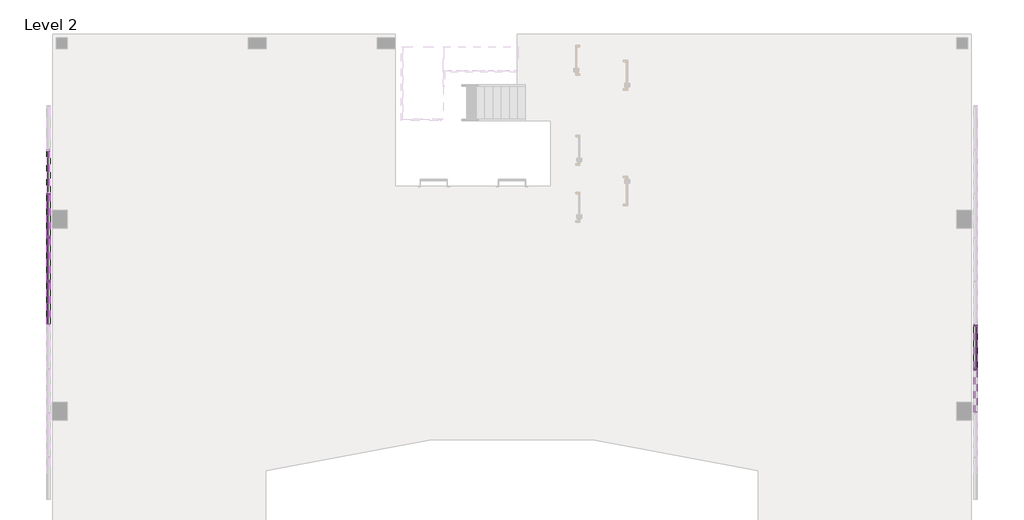
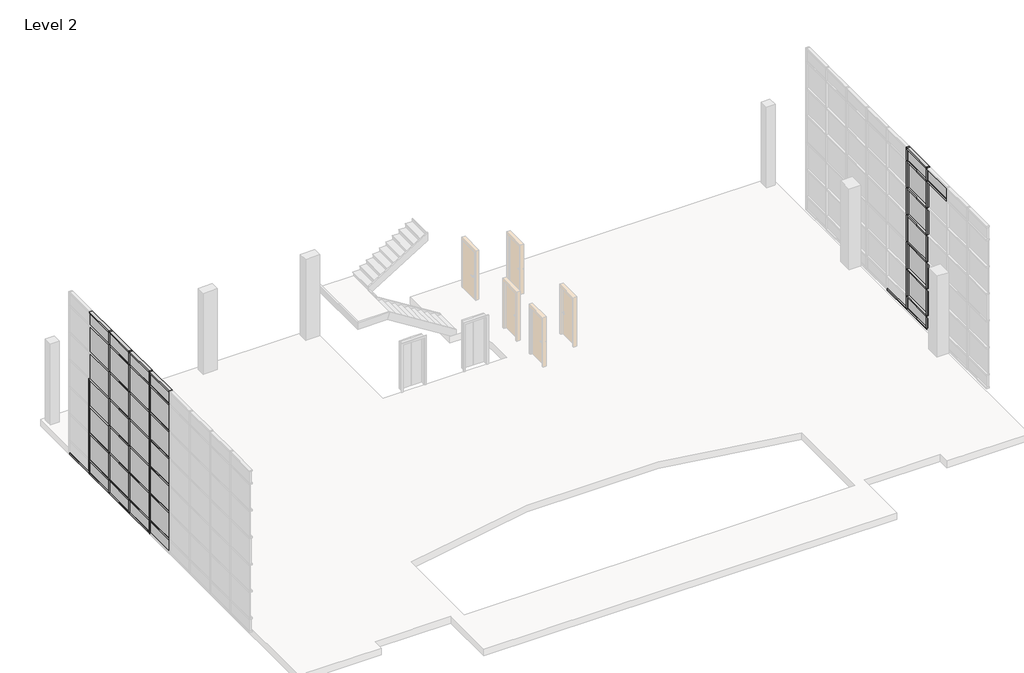
# One storey, part 4 of 6: 77 members, 36 plates.
"""IFC4 building model written with IfcOpenShell, lengths in millimetres."""

import ifcopenshell
import ifcopenshell.guid

model = None  # the IFC model being written
_history = None  # IfcOwnerHistory: only IFC2X3 demands one
_inside = {}  # id of a spatial element -> (the spatial element, [elements in it])
_under = {}  # id of a project, library or spatial element -> (it, [spatial elements below it])
_declared = {}  # id of a project -> (the project, [libraries it declares])
_typed = {}  # id of a type object -> (the type object, [elements of that type])
_made_of = {}  # id of a material, layer set ... -> (it, [elements and type objects made of it])


def new_model(schema):
    """Start an empty IFC model of exactly this schema.

    Asked for "IFC4X3", IfcOpenShell would pick the latest addendum, in which some entities
    have other attributes; the version numbers below select the first issue.
    IFC2X3 requires an IfcOwnerHistory on every rooted entity: one is made here for all.
    """
    global model, _history
    if schema == "IFC4X3":
        model = ifcopenshell.file(schema_version=(4, 3, 0, 0))
    else:
        model = ifcopenshell.file(schema=schema)
    _inside.clear()
    _under.clear()
    _declared.clear()
    _typed.clear()
    _made_of.clear()
    _history = None
    if model.schema == "IFC2X3":
        org = make("IfcOrganization", Name="unknown")
        user = make(
            "IfcPersonAndOrganization",
            ThePerson=make("IfcPerson", FamilyName="unknown"),
            TheOrganization=org,
        )
        app = make(
            "IfcApplication",
            ApplicationDeveloper=org,
            Version="unknown",
            ApplicationFullName="unknown",
            ApplicationIdentifier="unknown",
        )
        _history = make(
            "IfcOwnerHistory",
            OwningUser=user,
            OwningApplication=app,
            ChangeAction="ADDED",
            CreationDate=0,
        )
    return model


def make(cls, **values):
    """One entity of the class cls with the attributes given. An attribute that is None is left unset."""
    return model.create_entity(
        cls, **{name: value for name, value in values.items() if value is not None}
    )


def rooted(cls, **values):
    """An entity with a GlobalId (a new one), such as an element, a storey or a relation."""
    return make(cls, GlobalId=ifcopenshell.guid.new(), OwnerHistory=_history, **values)


def si_unit(unit_type, name, prefix=None):
    """IfcSIUnit, for example si_unit("LENGTHUNIT", "METRE", prefix="MILLI")."""
    return make("IfcSIUnit", UnitType=unit_type, Prefix=prefix, Name=name)


def assignment(units):
    """IfcUnitAssignment: the units of a project."""
    return None if units is None else make("IfcUnitAssignment", Units=units)


def point(xyz):
    """IfcCartesianPoint."""
    return None if xyz is None else make("IfcCartesianPoint", Coordinates=xyz)


def direction(xyz):
    """IfcDirection."""
    return None if xyz is None else make("IfcDirection", DirectionRatios=xyz)


def frame(location, z_axis=None, x_axis=None):
    """IfcAxis2Placement3D, a coordinate frame: its origin and axes. An axis left out is left unset."""
    return make(
        "IfcAxis2Placement3D",
        Location=point(location),
        Axis=direction(z_axis),
        RefDirection=direction(x_axis),
    )


def origin():
    """The frame at (0, 0, 0) with its axes left unset."""
    return frame((0.0, 0.0, 0.0))


def origin_with_axes():
    """The frame at (0, 0, 0) with the z axis (0, 0, 1) and the x axis (1, 0, 0) written out."""
    return frame((0.0, 0.0, 0.0), z_axis=(0.0, 0.0, 1.0), x_axis=(1.0, 0.0, 0.0))


def place(relative_to, where):
    """IfcLocalPlacement: puts the frame where relative to a parent placement (None: the world)."""
    return make(
        "IfcLocalPlacement", PlacementRelTo=relative_to, RelativePlacement=where
    )


def context(
    kind, dimensions, precision=None, world=None, true_north=None, identifier=None
):
    """IfcGeometricRepresentationContext, for example the 3D "Model" context."""
    return make(
        "IfcGeometricRepresentationContext",
        ContextIdentifier=identifier,
        ContextType=kind,
        CoordinateSpaceDimension=dimensions,
        Precision=precision,
        WorldCoordinateSystem=world,
        TrueNorth=true_north,
    )


def project(units=None, contexts=None):
    """IfcProject with its units and contexts."""
    return rooted(
        "IfcProject",
        Name="project",
        RepresentationContexts=contexts,
        UnitsInContext=assignment(units),
    )


def spatial(cls, under=None, at=None, **own):
    """A site, building, storey or space (cls), placed at a placement, below another one or the project."""
    s = rooted(cls, ObjectPlacement=at, **own)
    if under is not None:
        _under.setdefault(under.id(), (under, []))[1].append(s)
    return s


def polyline(points):
    """IfcPolyline through the points."""
    return make("IfcPolyline", Points=[point(p) for p in points])


def outline(outer, holes=None, kind="AREA"):
    """IfcArbitraryClosedProfileDef: a profile drawn as a closed curve; with holes, ...WithVoids."""
    if holes is None:
        return make("IfcArbitraryClosedProfileDef", ProfileType=kind, OuterCurve=outer)
    return make(
        "IfcArbitraryProfileDefWithVoids",
        ProfileType=kind,
        OuterCurve=outer,
        InnerCurves=holes,
    )


def extrude(swept, where, along, depth):
    """IfcExtrudedAreaSolid: the profile swept, set in the frame where, extruded along a direction by depth."""
    return make(
        "IfcExtrudedAreaSolid",
        SweptArea=swept,
        Position=where,
        ExtrudedDirection=direction(along),
        Depth=depth,
    )


def shape(context_of_items, identifier, shape_type, items):
    """IfcShapeRepresentation: the items that make up one representation, for example the "Body"."""
    return make(
        "IfcShapeRepresentation",
        ContextOfItems=context_of_items,
        RepresentationIdentifier=identifier,
        RepresentationType=shape_type,
        Items=items,
    )


def source(mapping_origin, context_of_items, identifier, shape_type, items):
    """IfcRepresentationMap: a shape defined once, which mapped items show again and again."""
    return make(
        "IfcRepresentationMap",
        MappingOrigin=mapping_origin,
        MappedRepresentation=shape(context_of_items, identifier, shape_type, items),
    )


def transform(
    local_origin,
    x_axis=None,
    y_axis=None,
    z_axis=None,
    scale=None,
    scale2=None,
    scale3=None,
    uniform=True,
):
    """IfcCartesianTransformationOperator3D, or its non-uniform kind. x_axis, y_axis, z_axis: its Axis1, 2, 3."""
    if uniform:
        return make(
            "IfcCartesianTransformationOperator3D",
            Axis1=direction(x_axis),
            Axis2=direction(y_axis),
            LocalOrigin=point(local_origin),
            Scale=scale,
            Axis3=direction(z_axis),
        )
    return make(
        "IfcCartesianTransformationOperator3DnonUniform",
        Axis1=direction(x_axis),
        Axis2=direction(y_axis),
        LocalOrigin=point(local_origin),
        Scale=scale,
        Axis3=direction(z_axis),
        Scale2=scale2,
        Scale3=scale3,
    )


def mapped(mapping_source, mapping_target):
    """IfcMappedItem: shows the shape of a source again, moved by a transform."""
    return make(
        "IfcMappedItem", MappingSource=mapping_source, MappingTarget=mapping_target
    )


def made_of(thing, what):
    """Note that an element or type object is made of a material, layer set ...; save() writes the relation."""
    if what is not None:
        _made_of.setdefault(what.id(), (what, []))[1].append(thing)
    return thing


def element(
    cls,
    number,
    at=None,
    inside=None,
    cuts=None,
    type_object=None,
    material=None,
    context=None,
    identifier="Body",
    shape_type=None,
    held_by="IfcProductDefinitionShape",
    body=None,
    shapes=None,
    **own,
):
    """One element of the class cls, such as IfcWall. Its Tag is "e" and its number.

    at: its placement. inside: the storey or other place that contains it. cuts: it is an
    opening in that element (IfcRelVoidsElement). A single representation is given by context,
    identifier, shape_type and body (its items); several are given by shapes. held_by: the class
    of the entity that holds the representations. save() writes the other relations.
    """
    e = rooted(cls, Tag="e%d" % number, ObjectPlacement=at, **own)
    if body is not None:
        shapes = [shape(context, identifier, shape_type, body)]
    if shapes is not None:
        e.Representation = make(held_by, Representations=shapes)
    if inside is not None:
        _inside.setdefault(inside.id(), (inside, []))[1].append(e)
    if cuts is not None:
        rooted(
            "IfcRelVoidsElement", RelatingBuildingElement=cuts, RelatedOpeningElement=e
        )
    if type_object is not None:
        _typed.setdefault(type_object.id(), (type_object, []))[1].append(e)
    return made_of(e, material)


def aggregate(whole, parts):
    """IfcRelAggregates: a whole, such as a stair, and the parts it consists of."""
    return rooted("IfcRelAggregates", RelatingObject=whole, RelatedObjects=parts)


def save(model, path):
    """Write the relations noted so far, then the file.

    IfcRelAggregates (storeys below a building ...), IfcRelContainedInSpatialStructure (elements
    in a storey), IfcRelDefinesByType, IfcRelAssociatesMaterial and IfcRelDeclares: one each for
    every whole, place, type object, material and project.
    """
    for whole, parts in _under.values():
        aggregate(whole, parts)
    for where, things in _inside.values():
        rooted(
            "IfcRelContainedInSpatialStructure",
            RelatedElements=things,
            RelatingStructure=where,
        )
    for kind, things in _typed.values():
        rooted("IfcRelDefinesByType", RelatedObjects=things, RelatingType=kind)
    for what, things in _made_of.values():
        rooted("IfcRelAssociatesMaterial", RelatedObjects=things, RelatingMaterial=what)
    for by, libraries in _declared.values():
        rooted("IfcRelDeclares", RelatingContext=by, RelatedDefinitions=libraries)
    model.write(path)


def member_2e151cea(model_context):
    return source(origin(), model_context, "Body", "SweptSolid", [
        extrude(outline(polyline([(0.0, 63.5), (0.0, -63.5), (-63.5, -63.5), (-63.5, 63.5), (0.0, 63.5)])), frame((0.0, 0.0, -1426.6333333), z_axis=(0.0, 0.0, 1.0), x_axis=(1.0, 0.0, 0.0)), (0.0, 0.0, 1.0), 1426.6333333),
    ])


def member_7b0bb32c(model_context):
    return source(origin(), model_context, "Body", "SweptSolid", [
        extrude(outline(polyline([(0.0, 63.5), (0.0, -63.5), (-63.5, -63.5), (-63.5, 63.5), (0.0, 63.5)])), frame((0.0, 0.0, -1394.8833336), z_axis=(0.0, 0.0, 1.0), x_axis=(1.0, 0.0, 0.0)), (0.0, 0.0, 1.0), 1394.8833336),
    ])


def member_3c30aa5e(model_context):
    return source(origin(), model_context, "Body", "SweptSolid", [
        extrude(outline(polyline([(31.75, 63.5), (31.75, -63.5), (-31.75, -63.5), (-31.75, 63.5), (31.75, 63.5)])), frame((0.0, 0.0, -1426.6333333), z_axis=(0.0, 0.0, 1.0), x_axis=(1.0, 0.0, 0.0)), (0.0, 0.0, 1.0), 1426.6333333),
    ])


def member_2b49869a(model_context):
    return source(origin(), model_context, "Body", "SweptSolid", [
        extrude(outline(polyline([(31.75, 63.5), (31.75, -63.5), (-31.75, -63.5), (-31.75, 63.5), (31.75, 63.5)])), frame((0.0, 0.0, -1219.2), z_axis=(0.0, 0.0, 1.0), x_axis=(1.0, 0.0, 0.0)), (0.0, 0.0, 1.0), 1219.2),
    ])


def member_6e77e263(model_context):
    return source(origin(), model_context, "Body", "SweptSolid", [
        extrude(outline(polyline([(31.75, 63.5), (31.75, -63.5), (-31.75, -63.5), (-31.75, 63.5), (31.75, 63.5)])), frame((0.0, 0.0, -609.6), z_axis=(0.0, 0.0, 1.0), x_axis=(1.0, 0.0, 0.0)), (0.0, 0.0, 1.0), 609.6),
    ])


def system_panel_glazed_8e8b8cb0(model_context):
    return source(origin(), model_context, "Body", "SweptSolid", [
        extrude(outline(polyline([(713.3166666, 19.05), (-713.3166666, 19.05), (-713.3166666, 44.45), (713.3166666, 44.45), (713.3166666, 19.05)])), origin_with_axes(), (0.0, 0.0, 1.0), 1155.7),
    ])


def system_panel_glazed_0adb819a(model_context):
    return source(origin(), model_context, "Body", "SweptSolid", [
        extrude(outline(polyline([(713.3166666, -44.45), (-713.3166666, -44.45), (-713.3166666, -19.05), (713.3166666, -19.05), (713.3166666, -44.45)])), origin_with_axes(), (0.0, 0.0, 1.0), 1155.7),
    ])


def system_panel_solid_81e17396(model_context):
    return source(origin(), model_context, "Body", "SweptSolid", [
        extrude(outline(polyline([(713.3166666, -19.05), (-713.3166666, -19.05), (-713.3166666, 44.45), (713.3166666, 44.45), (713.3166666, -19.05)])), origin_with_axes(), (0.0, 0.0, 1.0), 1155.7),
    ])


def system_panel_solid_4932440a(model_context):
    return source(origin(), model_context, "Body", "SweptSolid", [
        extrude(outline(polyline([(713.3166666, -19.05), (-713.3166666, -19.05), (-713.3166666, 44.45), (713.3166666, 44.45), (713.3166666, -19.05)])), origin_with_axes(), (0.0, 0.0, 1.0), 514.35),
    ])


def system_panel_solid_81598777(model_context):
    return source(origin(), model_context, "Body", "SweptSolid", [
        extrude(outline(polyline([(713.3166666, -44.45), (-713.3166666, -44.45), (-713.3166666, 19.05), (713.3166666, 19.05), (713.3166666, -44.45)])), origin_with_axes(), (0.0, 0.0, 1.0), 514.35),
    ])


def system_panel_solid_db88bede(model_context):
    return source(origin(), model_context, "Body", "SweptSolid", [
        extrude(outline(polyline([(713.3166666, -44.45), (-713.3166666, -44.45), (-713.3166666, 19.05), (713.3166666, 19.05), (713.3166666, -44.45)])), origin_with_axes(), (0.0, 0.0, 1.0), 1155.7),
    ])


model = new_model("IFC4")

# Units and contexts
model_context = context("Model", 3, world=origin())
ifc_project = project(units=[si_unit("LENGTHUNIT", "METRE", prefix="MILLI")], contexts=[model_context])

# Site, building, storey
site = spatial("IfcSite", under=ifc_project)
building = spatial("IfcBuilding", under=site)
storey = spatial("IfcBuildingStorey", under=building, Name="Level 2", Elevation=3657.6)

# Members
placement = place(None, origin())
member_shape = member_2e151cea(model_context)
element("IfcMember", 1, ObjectType="Rectangular Mullion : 2.5\" x 5\" rectangular", at=placement, inside=storey, context=model_context, shape_type="MappedRepresentation", body=[
    mapped(member_shape, transform((-16888.4122732, 962.418197, 10972.8), x_axis=(0.0, 0.0, 1.0), y_axis=(1.0, 0.0, 0.0), z_axis=(0.0, 1.0, 0.0))),
])
element("IfcMember", 2, ObjectType="Rectangular Mullion : 2.5\" x 5\" rectangular", at=placement, inside=storey, context=model_context, shape_type="MappedRepresentation", body=[
    mapped(member_shape, transform((-16888.4122732, 2452.5515303, 10972.8), x_axis=(0.0, 0.0, 1.0), y_axis=(1.0, 0.0, 0.0), z_axis=(0.0, 1.0, 0.0))),
])
element("IfcMember", 3, ObjectType="Rectangular Mullion : 2.5\" x 5\" rectangular", at=placement, inside=storey, context=model_context, shape_type="MappedRepresentation", body=[
    mapped(member_shape, transform((-16888.4122732, 3942.6848636, 10972.8), x_axis=(0.0, 0.0, 1.0), y_axis=(1.0, 0.0, 0.0), z_axis=(0.0, 1.0, 0.0))),
])
element("IfcMember", 4, ObjectType="Rectangular Mullion : 2.5\" x 5\" rectangular", at=placement, inside=storey, context=model_context, shape_type="MappedRepresentation", body=[
    mapped(member_shape, transform((-16888.4122732, 5432.8181968, 10972.8), x_axis=(0.0, 0.0, 1.0), y_axis=(1.0, 0.0, 0.0), z_axis=(0.0, 1.0, 0.0))),
])
member_2_shape = member_7b0bb32c(model_context)
element("IfcMember", 5, ObjectType="Rectangular Mullion : 2.5\" x 5\" rectangular", at=placement, inside=storey, context=model_context, shape_type="MappedRepresentation", body=[
    mapped(member_2_shape, transform((-16888.4122732, 5496.3181968, 3657.6), x_axis=(0.0, 0.0, -1.0), y_axis=(1.0, 0.0, 0.0), z_axis=(0.0, -1.0, 0.0))),
])
element("IfcMember", 6, ObjectType="Rectangular Mullion : 2.5\" x 5\" rectangular", at=placement, inside=storey, context=model_context, shape_type="MappedRepresentation", body=[
    mapped(member_shape, transform((-16888.4122732, 1025.918197, 3657.6), x_axis=(0.0, 0.0, -1.0), y_axis=(1.0, 0.0, 0.0), z_axis=(0.0, -1.0, 0.0))),
])
element("IfcMember", 7, ObjectType="Rectangular Mullion : 2.5\" x 5\" rectangular", at=placement, inside=storey, context=model_context, shape_type="MappedRepresentation", body=[
    mapped(member_shape, transform((-16888.4122732, 2516.0515303, 3657.6), x_axis=(0.0, 0.0, -1.0), y_axis=(1.0, 0.0, 0.0), z_axis=(0.0, -1.0, 0.0))),
])
element("IfcMember", 8, ObjectType="Rectangular Mullion : 2.5\" x 5\" rectangular", at=placement, inside=storey, context=model_context, shape_type="MappedRepresentation", body=[
    mapped(member_shape, transform((-16888.4122732, 4006.1848636, 3657.6), x_axis=(0.0, 0.0, -1.0), y_axis=(1.0, 0.0, 0.0), z_axis=(0.0, -1.0, 0.0))),
])
member_3_shape = member_3c30aa5e(model_context)
element("IfcMember", 9, ObjectType="Rectangular Mullion : 2.5\" x 5\" rectangular", at=placement, inside=storey, context=model_context, shape_type="MappedRepresentation", body=[
    mapped(member_3_shape, transform((-16888.4122732, 962.418197, 4267.2), x_axis=(0.0, 0.0, 1.0), y_axis=(1.0, 0.0, 0.0), z_axis=(0.0, 1.0, 0.0))),
])
element("IfcMember", 10, ObjectType="Rectangular Mullion : 2.5\" x 5\" rectangular", at=placement, inside=storey, context=model_context, shape_type="MappedRepresentation", body=[
    mapped(member_3_shape, transform((-16888.4122732, 2452.5515303, 4267.2), x_axis=(0.0, 0.0, 1.0), y_axis=(1.0, 0.0, 0.0), z_axis=(0.0, 1.0, 0.0))),
])
element("IfcMember", 11, ObjectType="Rectangular Mullion : 2.5\" x 5\" rectangular", at=placement, inside=storey, context=model_context, shape_type="MappedRepresentation", body=[
    mapped(member_3_shape, transform((-16888.4122732, 3942.6848636, 4267.2), x_axis=(0.0, 0.0, 1.0), y_axis=(1.0, 0.0, 0.0), z_axis=(0.0, 1.0, 0.0))),
])
element("IfcMember", 12, ObjectType="Rectangular Mullion : 2.5\" x 5\" rectangular", at=placement, inside=storey, context=model_context, shape_type="MappedRepresentation", body=[
    mapped(member_3_shape, transform((-16888.4122732, 5432.8181968, 4267.2), x_axis=(0.0, 0.0, 1.0), y_axis=(1.0, 0.0, 0.0), z_axis=(0.0, 1.0, 0.0))),
])
element("IfcMember", 13, ObjectType="Rectangular Mullion : 2.5\" x 5\" rectangular", at=placement, inside=storey, context=model_context, shape_type="MappedRepresentation", body=[
    mapped(member_3_shape, transform((-16888.4122732, 962.418197, 5486.4), x_axis=(0.0, 0.0, 1.0), y_axis=(1.0, 0.0, 0.0), z_axis=(0.0, 1.0, 0.0))),
])
element("IfcMember", 14, ObjectType="Rectangular Mullion : 2.5\" x 5\" rectangular", at=placement, inside=storey, context=model_context, shape_type="MappedRepresentation", body=[
    mapped(member_3_shape, transform((-16888.4122732, 2452.5515303, 5486.4), x_axis=(0.0, 0.0, 1.0), y_axis=(1.0, 0.0, 0.0), z_axis=(0.0, 1.0, 0.0))),
])
element("IfcMember", 15, ObjectType="Rectangular Mullion : 2.5\" x 5\" rectangular", at=placement, inside=storey, context=model_context, shape_type="MappedRepresentation", body=[
    mapped(member_3_shape, transform((-16888.4122732, 3942.6848636, 5486.4), x_axis=(0.0, 0.0, 1.0), y_axis=(1.0, 0.0, 0.0), z_axis=(0.0, 1.0, 0.0))),
])
element("IfcMember", 16, ObjectType="Rectangular Mullion : 2.5\" x 5\" rectangular", at=placement, inside=storey, context=model_context, shape_type="MappedRepresentation", body=[
    mapped(member_3_shape, transform((-16888.4122732, 5432.8181968, 5486.4), x_axis=(0.0, 0.0, 1.0), y_axis=(1.0, 0.0, 0.0), z_axis=(0.0, 1.0, 0.0))),
])
element("IfcMember", 17, ObjectType="Rectangular Mullion : 2.5\" x 5\" rectangular", at=placement, inside=storey, context=model_context, shape_type="MappedRepresentation", body=[
    mapped(member_3_shape, transform((-16888.4122732, 962.418197, 6705.6), x_axis=(0.0, 0.0, 1.0), y_axis=(1.0, 0.0, 0.0), z_axis=(0.0, 1.0, 0.0))),
])
element("IfcMember", 18, ObjectType="Rectangular Mullion : 2.5\" x 5\" rectangular", at=placement, inside=storey, context=model_context, shape_type="MappedRepresentation", body=[
    mapped(member_3_shape, transform((-16888.4122732, 2452.5515303, 6705.6), x_axis=(0.0, 0.0, 1.0), y_axis=(1.0, 0.0, 0.0), z_axis=(0.0, 1.0, 0.0))),
])
element("IfcMember", 19, ObjectType="Rectangular Mullion : 2.5\" x 5\" rectangular", at=placement, inside=storey, context=model_context, shape_type="MappedRepresentation", body=[
    mapped(member_3_shape, transform((-16888.4122732, 3942.6848636, 6705.6), x_axis=(0.0, 0.0, 1.0), y_axis=(1.0, 0.0, 0.0), z_axis=(0.0, 1.0, 0.0))),
])
element("IfcMember", 20, ObjectType="Rectangular Mullion : 2.5\" x 5\" rectangular", at=placement, inside=storey, context=model_context, shape_type="MappedRepresentation", body=[
    mapped(member_3_shape, transform((-16888.4122732, 962.418197, 7924.8), x_axis=(0.0, 0.0, 1.0), y_axis=(1.0, 0.0, 0.0), z_axis=(0.0, 1.0, 0.0))),
])
element("IfcMember", 21, ObjectType="Rectangular Mullion : 2.5\" x 5\" rectangular", at=placement, inside=storey, context=model_context, shape_type="MappedRepresentation", body=[
    mapped(member_3_shape, transform((-16888.4122732, 2452.5515303, 7924.8), x_axis=(0.0, 0.0, 1.0), y_axis=(1.0, 0.0, 0.0), z_axis=(0.0, 1.0, 0.0))),
])
element("IfcMember", 22, ObjectType="Rectangular Mullion : 2.5\" x 5\" rectangular", at=placement, inside=storey, context=model_context, shape_type="MappedRepresentation", body=[
    mapped(member_3_shape, transform((-16888.4122732, 3942.6848636, 7924.8), x_axis=(0.0, 0.0, 1.0), y_axis=(1.0, 0.0, 0.0), z_axis=(0.0, 1.0, 0.0))),
])
element("IfcMember", 23, ObjectType="Rectangular Mullion : 2.5\" x 5\" rectangular", at=placement, inside=storey, context=model_context, shape_type="MappedRepresentation", body=[
    mapped(member_3_shape, transform((-16888.4122732, 962.418197, 9144.0), x_axis=(0.0, 0.0, 1.0), y_axis=(1.0, 0.0, 0.0), z_axis=(0.0, 1.0, 0.0))),
])
element("IfcMember", 24, ObjectType="Rectangular Mullion : 2.5\" x 5\" rectangular", at=placement, inside=storey, context=model_context, shape_type="MappedRepresentation", body=[
    mapped(member_3_shape, transform((-16888.4122732, 2452.5515303, 9144.0), x_axis=(0.0, 0.0, 1.0), y_axis=(1.0, 0.0, 0.0), z_axis=(0.0, 1.0, 0.0))),
])
element("IfcMember", 25, ObjectType="Rectangular Mullion : 2.5\" x 5\" rectangular", at=placement, inside=storey, context=model_context, shape_type="MappedRepresentation", body=[
    mapped(member_3_shape, transform((-16888.4122732, 3942.6848636, 9144.0), x_axis=(0.0, 0.0, 1.0), y_axis=(1.0, 0.0, 0.0), z_axis=(0.0, 1.0, 0.0))),
])
element("IfcMember", 26, ObjectType="Rectangular Mullion : 2.5\" x 5\" rectangular", at=placement, inside=storey, context=model_context, shape_type="MappedRepresentation", body=[
    mapped(member_3_shape, transform((-16888.4122732, 962.418197, 10363.2), x_axis=(0.0, 0.0, 1.0), y_axis=(1.0, 0.0, 0.0), z_axis=(0.0, 1.0, 0.0))),
])
element("IfcMember", 27, ObjectType="Rectangular Mullion : 2.5\" x 5\" rectangular", at=placement, inside=storey, context=model_context, shape_type="MappedRepresentation", body=[
    mapped(member_3_shape, transform((-16888.4122732, 2452.5515303, 10363.2), x_axis=(0.0, 0.0, 1.0), y_axis=(1.0, 0.0, 0.0), z_axis=(0.0, 1.0, 0.0))),
])
element("IfcMember", 28, ObjectType="Rectangular Mullion : 2.5\" x 5\" rectangular", at=placement, inside=storey, context=model_context, shape_type="MappedRepresentation", body=[
    mapped(member_3_shape, transform((-16888.4122732, 3942.6848636, 10363.2), x_axis=(0.0, 0.0, 1.0), y_axis=(1.0, 0.0, 0.0), z_axis=(0.0, 1.0, 0.0))),
])
member_4_shape = member_2b49869a(model_context)
element("IfcMember", 29, ObjectType="Rectangular Mullion : 2.5\" x 5\" rectangular", at=placement, inside=storey, context=model_context, shape_type="MappedRepresentation", body=[
    mapped(member_4_shape, transform((-16888.4122732, 994.168197, 4267.2), x_axis=(0.0, 1.0, 0.0), y_axis=(1.0, 0.0, 0.0), z_axis=(0.0, 0.0, -1.0))),
])
element("IfcMember", 30, ObjectType="Rectangular Mullion : 2.5\" x 5\" rectangular", at=placement, inside=storey, context=model_context, shape_type="MappedRepresentation", body=[
    mapped(member_4_shape, transform((-16888.4122732, 2484.3015303, 4267.2), x_axis=(0.0, 1.0, 0.0), y_axis=(1.0, 0.0, 0.0), z_axis=(0.0, 0.0, -1.0))),
])
element("IfcMember", 31, ObjectType="Rectangular Mullion : 2.5\" x 5\" rectangular", at=placement, inside=storey, context=model_context, shape_type="MappedRepresentation", body=[
    mapped(member_4_shape, transform((-16888.4122732, 3974.4348636, 4267.2), x_axis=(0.0, 1.0, 0.0), y_axis=(1.0, 0.0, 0.0), z_axis=(0.0, 0.0, -1.0))),
])
element("IfcMember", 32, ObjectType="Rectangular Mullion : 2.5\" x 5\" rectangular", at=placement, inside=storey, context=model_context, shape_type="MappedRepresentation", body=[
    mapped(member_4_shape, transform((-16888.4122732, 5464.5681968, 4267.2), x_axis=(0.0, 1.0, 0.0), y_axis=(1.0, 0.0, 0.0), z_axis=(0.0, 0.0, -1.0))),
])
element("IfcMember", 33, ObjectType="Rectangular Mullion : 2.5\" x 5\" rectangular", at=placement, inside=storey, context=model_context, shape_type="MappedRepresentation", body=[
    mapped(member_4_shape, transform((-16888.4122732, 994.168197, 5486.4), x_axis=(0.0, 1.0, 0.0), y_axis=(1.0, 0.0, 0.0), z_axis=(0.0, 0.0, -1.0))),
])
element("IfcMember", 34, ObjectType="Rectangular Mullion : 2.5\" x 5\" rectangular", at=placement, inside=storey, context=model_context, shape_type="MappedRepresentation", body=[
    mapped(member_4_shape, transform((-16888.4122732, 2484.3015303, 5486.4), x_axis=(0.0, 1.0, 0.0), y_axis=(1.0, 0.0, 0.0), z_axis=(0.0, 0.0, -1.0))),
])
element("IfcMember", 35, ObjectType="Rectangular Mullion : 2.5\" x 5\" rectangular", at=placement, inside=storey, context=model_context, shape_type="MappedRepresentation", body=[
    mapped(member_4_shape, transform((-16888.4122732, 3974.4348636, 5486.4), x_axis=(0.0, 1.0, 0.0), y_axis=(1.0, 0.0, 0.0), z_axis=(0.0, 0.0, -1.0))),
])
element("IfcMember", 36, ObjectType="Rectangular Mullion : 2.5\" x 5\" rectangular", at=placement, inside=storey, context=model_context, shape_type="MappedRepresentation", body=[
    mapped(member_4_shape, transform((-16888.4122732, 5464.5681968, 5486.4), x_axis=(0.0, 1.0, 0.0), y_axis=(1.0, 0.0, 0.0), z_axis=(0.0, 0.0, -1.0))),
])
element("IfcMember", 37, ObjectType="Rectangular Mullion : 2.5\" x 5\" rectangular", at=placement, inside=storey, context=model_context, shape_type="MappedRepresentation", body=[
    mapped(member_4_shape, transform((-16888.4122732, 994.168197, 6705.6), x_axis=(0.0, 1.0, 0.0), y_axis=(1.0, 0.0, 0.0), z_axis=(0.0, 0.0, -1.0))),
])
element("IfcMember", 38, ObjectType="Rectangular Mullion : 2.5\" x 5\" rectangular", at=placement, inside=storey, context=model_context, shape_type="MappedRepresentation", body=[
    mapped(member_4_shape, transform((-16888.4122732, 994.168197, 7924.8), x_axis=(0.0, 1.0, 0.0), y_axis=(1.0, 0.0, 0.0), z_axis=(0.0, 0.0, -1.0))),
])
element("IfcMember", 39, ObjectType="Rectangular Mullion : 2.5\" x 5\" rectangular", at=placement, inside=storey, context=model_context, shape_type="MappedRepresentation", body=[
    mapped(member_4_shape, transform((-16888.4122732, 994.168197, 9144.0), x_axis=(0.0, 1.0, 0.0), y_axis=(1.0, 0.0, 0.0), z_axis=(0.0, 0.0, -1.0))),
])
element("IfcMember", 40, ObjectType="Rectangular Mullion : 2.5\" x 5\" rectangular", at=placement, inside=storey, context=model_context, shape_type="MappedRepresentation", body=[
    mapped(member_4_shape, transform((-16888.4122732, 2484.3015303, 6705.6), x_axis=(0.0, 1.0, 0.0), y_axis=(1.0, 0.0, 0.0), z_axis=(0.0, 0.0, -1.0))),
])
element("IfcMember", 41, ObjectType="Rectangular Mullion : 2.5\" x 5\" rectangular", at=placement, inside=storey, context=model_context, shape_type="MappedRepresentation", body=[
    mapped(member_4_shape, transform((-16888.4122732, 2484.3015303, 7924.8), x_axis=(0.0, 1.0, 0.0), y_axis=(1.0, 0.0, 0.0), z_axis=(0.0, 0.0, -1.0))),
])
element("IfcMember", 42, ObjectType="Rectangular Mullion : 2.5\" x 5\" rectangular", at=placement, inside=storey, context=model_context, shape_type="MappedRepresentation", body=[
    mapped(member_4_shape, transform((-16888.4122732, 2484.3015303, 9144.0), x_axis=(0.0, 1.0, 0.0), y_axis=(1.0, 0.0, 0.0), z_axis=(0.0, 0.0, -1.0))),
])
element("IfcMember", 43, ObjectType="Rectangular Mullion : 2.5\" x 5\" rectangular", at=placement, inside=storey, context=model_context, shape_type="MappedRepresentation", body=[
    mapped(member_4_shape, transform((-16888.4122732, 3974.4348636, 6705.6), x_axis=(0.0, 1.0, 0.0), y_axis=(1.0, 0.0, 0.0), z_axis=(0.0, 0.0, -1.0))),
])
element("IfcMember", 44, ObjectType="Rectangular Mullion : 2.5\" x 5\" rectangular", at=placement, inside=storey, context=model_context, shape_type="MappedRepresentation", body=[
    mapped(member_4_shape, transform((-16888.4122732, 3974.4348636, 7924.8), x_axis=(0.0, 1.0, 0.0), y_axis=(1.0, 0.0, 0.0), z_axis=(0.0, 0.0, -1.0))),
])
element("IfcMember", 45, ObjectType="Rectangular Mullion : 2.5\" x 5\" rectangular", at=placement, inside=storey, context=model_context, shape_type="MappedRepresentation", body=[
    mapped(member_4_shape, transform((-16888.4122732, 3974.4348636, 9144.0), x_axis=(0.0, 1.0, 0.0), y_axis=(1.0, 0.0, 0.0), z_axis=(0.0, 0.0, -1.0))),
])
element("IfcMember", 46, ObjectType="Rectangular Mullion : 2.5\" x 5\" rectangular", at=placement, inside=storey, context=model_context, shape_type="MappedRepresentation", body=[
    mapped(member_4_shape, transform((-16888.4122732, 5464.5681968, 6705.6), x_axis=(0.0, 1.0, 0.0), y_axis=(1.0, 0.0, 0.0), z_axis=(0.0, 0.0, -1.0))),
])
member_5_shape = member_6e77e263(model_context)
element("IfcMember", 47, ObjectType="Rectangular Mullion : 2.5\" x 5\" rectangular", at=placement, inside=storey, context=model_context, shape_type="MappedRepresentation", body=[
    mapped(member_5_shape, transform((-16888.4122732, 994.168197, 3657.6), x_axis=(0.0, 1.0, 0.0), y_axis=(1.0, 0.0, 0.0), z_axis=(0.0, 0.0, -1.0))),
])
element("IfcMember", 48, ObjectType="Rectangular Mullion : 2.5\" x 5\" rectangular", at=placement, inside=storey, context=model_context, shape_type="MappedRepresentation", body=[
    mapped(member_5_shape, transform((-16888.4122732, 2484.3015303, 3657.6), x_axis=(0.0, 1.0, 0.0), y_axis=(1.0, 0.0, 0.0), z_axis=(0.0, 0.0, -1.0))),
])
element("IfcMember", 49, ObjectType="Rectangular Mullion : 2.5\" x 5\" rectangular", at=placement, inside=storey, context=model_context, shape_type="MappedRepresentation", body=[
    mapped(member_5_shape, transform((-16888.4122732, 3974.4348636, 3657.6), x_axis=(0.0, 1.0, 0.0), y_axis=(1.0, 0.0, 0.0), z_axis=(0.0, 0.0, -1.0))),
])
element("IfcMember", 50, ObjectType="Rectangular Mullion : 2.5\" x 5\" rectangular", at=placement, inside=storey, context=model_context, shape_type="MappedRepresentation", body=[
    mapped(member_5_shape, transform((-16888.4122732, 5464.5681968, 3657.6), x_axis=(0.0, 1.0, 0.0), y_axis=(1.0, 0.0, 0.0), z_axis=(0.0, 0.0, -1.0))),
])
element("IfcMember", 51, ObjectType="Rectangular Mullion : 2.5\" x 5\" rectangular", at=placement, inside=storey, context=model_context, shape_type="MappedRepresentation", body=[
    mapped(member_5_shape, transform((-16888.4122732, 994.168197, 10363.2), x_axis=(0.0, 1.0, 0.0), y_axis=(1.0, 0.0, 0.0), z_axis=(0.0, 0.0, -1.0))),
])
element("IfcMember", 52, ObjectType="Rectangular Mullion : 2.5\" x 5\" rectangular", at=placement, inside=storey, context=model_context, shape_type="MappedRepresentation", body=[
    mapped(member_5_shape, transform((-16888.4122732, 2484.3015303, 10363.2), x_axis=(0.0, 1.0, 0.0), y_axis=(1.0, 0.0, 0.0), z_axis=(0.0, 0.0, -1.0))),
])
element("IfcMember", 53, ObjectType="Rectangular Mullion : 2.5\" x 5\" rectangular", at=placement, inside=storey, context=model_context, shape_type="MappedRepresentation", body=[
    mapped(member_5_shape, transform((-16888.4122732, 3974.4348636, 10363.2), x_axis=(0.0, 1.0, 0.0), y_axis=(1.0, 0.0, 0.0), z_axis=(0.0, 0.0, -1.0))),
])
element("IfcMember", 54, ObjectType="Rectangular Mullion : 2.5\" x 5\" rectangular", at=placement, inside=storey, context=model_context, shape_type="MappedRepresentation", body=[
    mapped(member_shape, transform((14556.9638541, -527.7151362, 10972.8), x_axis=(0.0, 0.0, 1.0), y_axis=(1.0, 0.0, 0.0), z_axis=(0.0, 1.0, 0.0))),
])
element("IfcMember", 55, ObjectType="Rectangular Mullion : 2.5\" x 5\" rectangular", at=placement, inside=storey, context=model_context, shape_type="MappedRepresentation", body=[
    mapped(member_shape, transform((14556.9638541, -1954.3484695, 3657.6), x_axis=(0.0, 0.0, -1.0), y_axis=(1.0, 0.0, 0.0), z_axis=(0.0, -1.0, 0.0))),
])
element("IfcMember", 56, ObjectType="Rectangular Mullion : 2.5\" x 5\" rectangular", at=placement, inside=storey, context=model_context, shape_type="MappedRepresentation", body=[
    mapped(member_shape, transform((14556.9638541, -464.2151362, 3657.6), x_axis=(0.0, 0.0, -1.0), y_axis=(1.0, 0.0, 0.0), z_axis=(0.0, -1.0, 0.0))),
])
element("IfcMember", 57, ObjectType="Rectangular Mullion : 2.5\" x 5\" rectangular", at=placement, inside=storey, context=model_context, shape_type="MappedRepresentation", body=[
    mapped(member_3_shape, transform((14556.9638541, -527.7151362, 4267.2), x_axis=(0.0, 0.0, 1.0), y_axis=(1.0, 0.0, 0.0), z_axis=(0.0, 1.0, 0.0))),
])
element("IfcMember", 58, ObjectType="Rectangular Mullion : 2.5\" x 5\" rectangular", at=placement, inside=storey, context=model_context, shape_type="MappedRepresentation", body=[
    mapped(member_3_shape, transform((14556.9638541, -527.7151362, 5486.4), x_axis=(0.0, 0.0, 1.0), y_axis=(1.0, 0.0, 0.0), z_axis=(0.0, 1.0, 0.0))),
])
element("IfcMember", 59, ObjectType="Rectangular Mullion : 2.5\" x 5\" rectangular", at=placement, inside=storey, context=model_context, shape_type="MappedRepresentation", body=[
    mapped(member_3_shape, transform((14556.9638541, -527.7151362, 6705.6), x_axis=(0.0, 0.0, 1.0), y_axis=(1.0, 0.0, 0.0), z_axis=(0.0, 1.0, 0.0))),
])
element("IfcMember", 60, ObjectType="Rectangular Mullion : 2.5\" x 5\" rectangular", at=placement, inside=storey, context=model_context, shape_type="MappedRepresentation", body=[
    mapped(member_3_shape, transform((14556.9638541, -527.7151362, 7924.8), x_axis=(0.0, 0.0, 1.0), y_axis=(1.0, 0.0, 0.0), z_axis=(0.0, 1.0, 0.0))),
])
element("IfcMember", 61, ObjectType="Rectangular Mullion : 2.5\" x 5\" rectangular", at=placement, inside=storey, context=model_context, shape_type="MappedRepresentation", body=[
    mapped(member_3_shape, transform((14556.9638541, -527.7151362, 9144.0), x_axis=(0.0, 0.0, 1.0), y_axis=(1.0, 0.0, 0.0), z_axis=(0.0, 1.0, 0.0))),
])
element("IfcMember", 62, ObjectType="Rectangular Mullion : 2.5\" x 5\" rectangular", at=placement, inside=storey, context=model_context, shape_type="MappedRepresentation", body=[
    mapped(member_3_shape, transform((14556.9638541, -2017.8484695, 10363.2), x_axis=(0.0, 0.0, 1.0), y_axis=(1.0, 0.0, 0.0), z_axis=(0.0, 1.0, 0.0))),
])
element("IfcMember", 63, ObjectType="Rectangular Mullion : 2.5\" x 5\" rectangular", at=placement, inside=storey, context=model_context, shape_type="MappedRepresentation", body=[
    mapped(member_3_shape, transform((14556.9638541, -527.7151362, 10363.2), x_axis=(0.0, 0.0, 1.0), y_axis=(1.0, 0.0, 0.0), z_axis=(0.0, 1.0, 0.0))),
])
element("IfcMember", 64, ObjectType="Rectangular Mullion : 2.5\" x 5\" rectangular", at=placement, inside=storey, context=model_context, shape_type="MappedRepresentation", body=[
    mapped(member_5_shape, transform((14556.9638541, -1986.0984695, 3657.6), x_axis=(0.0, 1.0, 0.0), y_axis=(1.0, 0.0, 0.0), z_axis=(0.0, 0.0, -1.0))),
])
element("IfcMember", 65, ObjectType="Rectangular Mullion : 2.5\" x 5\" rectangular", at=placement, inside=storey, context=model_context, shape_type="MappedRepresentation", body=[
    mapped(member_5_shape, transform((14556.9638541, -495.9651362, 3657.6), x_axis=(0.0, 1.0, 0.0), y_axis=(1.0, 0.0, 0.0), z_axis=(0.0, 0.0, -1.0))),
])
element("IfcMember", 66, ObjectType="Rectangular Mullion : 2.5\" x 5\" rectangular", at=placement, inside=storey, context=model_context, shape_type="MappedRepresentation", body=[
    mapped(member_4_shape, transform((14556.9638541, -1986.0984695, 4267.2), x_axis=(0.0, 1.0, 0.0), y_axis=(1.0, 0.0, 0.0), z_axis=(0.0, 0.0, -1.0))),
])
element("IfcMember", 67, ObjectType="Rectangular Mullion : 2.5\" x 5\" rectangular", at=placement, inside=storey, context=model_context, shape_type="MappedRepresentation", body=[
    mapped(member_4_shape, transform((14556.9638541, -495.9651362, 4267.2), x_axis=(0.0, 1.0, 0.0), y_axis=(1.0, 0.0, 0.0), z_axis=(0.0, 0.0, -1.0))),
])
element("IfcMember", 68, ObjectType="Rectangular Mullion : 2.5\" x 5\" rectangular", at=placement, inside=storey, context=model_context, shape_type="MappedRepresentation", body=[
    mapped(member_4_shape, transform((14556.9638541, -1986.0984695, 5486.4), x_axis=(0.0, 1.0, 0.0), y_axis=(1.0, 0.0, 0.0), z_axis=(0.0, 0.0, -1.0))),
])
element("IfcMember", 69, ObjectType="Rectangular Mullion : 2.5\" x 5\" rectangular", at=placement, inside=storey, context=model_context, shape_type="MappedRepresentation", body=[
    mapped(member_4_shape, transform((14556.9638541, -495.9651362, 5486.4), x_axis=(0.0, 1.0, 0.0), y_axis=(1.0, 0.0, 0.0), z_axis=(0.0, 0.0, -1.0))),
])
element("IfcMember", 70, ObjectType="Rectangular Mullion : 2.5\" x 5\" rectangular", at=placement, inside=storey, context=model_context, shape_type="MappedRepresentation", body=[
    mapped(member_4_shape, transform((14556.9638541, -1986.0984695, 6705.6), x_axis=(0.0, 1.0, 0.0), y_axis=(1.0, 0.0, 0.0), z_axis=(0.0, 0.0, -1.0))),
])
element("IfcMember", 71, ObjectType="Rectangular Mullion : 2.5\" x 5\" rectangular", at=placement, inside=storey, context=model_context, shape_type="MappedRepresentation", body=[
    mapped(member_4_shape, transform((14556.9638541, -1986.0984695, 7924.8), x_axis=(0.0, 1.0, 0.0), y_axis=(1.0, 0.0, 0.0), z_axis=(0.0, 0.0, -1.0))),
])
element("IfcMember", 72, ObjectType="Rectangular Mullion : 2.5\" x 5\" rectangular", at=placement, inside=storey, context=model_context, shape_type="MappedRepresentation", body=[
    mapped(member_4_shape, transform((14556.9638541, -1986.0984695, 9144.0), x_axis=(0.0, 1.0, 0.0), y_axis=(1.0, 0.0, 0.0), z_axis=(0.0, 0.0, -1.0))),
])
element("IfcMember", 73, ObjectType="Rectangular Mullion : 2.5\" x 5\" rectangular", at=placement, inside=storey, context=model_context, shape_type="MappedRepresentation", body=[
    mapped(member_4_shape, transform((14556.9638541, -495.9651362, 6705.6), x_axis=(0.0, 1.0, 0.0), y_axis=(1.0, 0.0, 0.0), z_axis=(0.0, 0.0, -1.0))),
])
element("IfcMember", 74, ObjectType="Rectangular Mullion : 2.5\" x 5\" rectangular", at=placement, inside=storey, context=model_context, shape_type="MappedRepresentation", body=[
    mapped(member_4_shape, transform((14556.9638541, -495.9651362, 7924.8), x_axis=(0.0, 1.0, 0.0), y_axis=(1.0, 0.0, 0.0), z_axis=(0.0, 0.0, -1.0))),
])
element("IfcMember", 75, ObjectType="Rectangular Mullion : 2.5\" x 5\" rectangular", at=placement, inside=storey, context=model_context, shape_type="MappedRepresentation", body=[
    mapped(member_4_shape, transform((14556.9638541, -495.9651362, 9144.0), x_axis=(0.0, 1.0, 0.0), y_axis=(1.0, 0.0, 0.0), z_axis=(0.0, 0.0, -1.0))),
])
element("IfcMember", 76, ObjectType="Rectangular Mullion : 2.5\" x 5\" rectangular", at=placement, inside=storey, context=model_context, shape_type="MappedRepresentation", body=[
    mapped(member_5_shape, transform((14556.9638541, -1986.0984695, 10363.2), x_axis=(0.0, 1.0, 0.0), y_axis=(1.0, 0.0, 0.0), z_axis=(0.0, 0.0, -1.0))),
])
element("IfcMember", 77, ObjectType="Rectangular Mullion : 2.5\" x 5\" rectangular", at=placement, inside=storey, context=model_context, shape_type="MappedRepresentation", body=[
    mapped(member_5_shape, transform((14556.9638541, -495.9651362, 10363.2), x_axis=(0.0, 1.0, 0.0), y_axis=(1.0, 0.0, 0.0), z_axis=(0.0, 0.0, -1.0))),
])

# Plates
system_panel_glazed_shape = system_panel_glazed_8e8b8cb0(model_context)
element("IfcPlate", 78, ObjectType="System Panel : Glazed", at=placement, inside=storey, context=model_context, shape_type="MappedRepresentation", body=[
    mapped(system_panel_glazed_shape, transform((-16888.4122732, 249.1015304, 4298.95), x_axis=(0.0, 1.0, 0.0), y_axis=(-1.0, 0.0, 0.0), z_axis=(0.0, 0.0, 1.0))),
])
element("IfcPlate", 79, ObjectType="System Panel : Glazed", at=placement, inside=storey, context=model_context, shape_type="MappedRepresentation", body=[
    mapped(system_panel_glazed_shape, transform((-16888.4122732, 1739.2348637, 4298.95), x_axis=(0.0, 1.0, 0.0), y_axis=(-1.0, 0.0, 0.0), z_axis=(0.0, 0.0, 1.0))),
])
element("IfcPlate", 80, ObjectType="System Panel : Glazed", at=placement, inside=storey, context=model_context, shape_type="MappedRepresentation", body=[
    mapped(system_panel_glazed_shape, transform((-16888.4122732, 3229.3681969, 4298.95), x_axis=(0.0, 1.0, 0.0), y_axis=(-1.0, 0.0, 0.0), z_axis=(0.0, 0.0, 1.0))),
])
element("IfcPlate", 81, ObjectType="System Panel : Glazed", at=placement, inside=storey, context=model_context, shape_type="MappedRepresentation", body=[
    mapped(system_panel_glazed_shape, transform((-16888.4122732, 4719.5015302, 4298.95), x_axis=(0.0, 1.0, 0.0), y_axis=(-1.0, 0.0, 0.0), z_axis=(0.0, 0.0, 1.0))),
])
element("IfcPlate", 82, ObjectType="System Panel : Glazed", at=placement, inside=storey, context=model_context, shape_type="MappedRepresentation", body=[
    mapped(system_panel_glazed_shape, transform((-16888.4122732, 249.1015304, 5518.15), x_axis=(0.0, 1.0, 0.0), y_axis=(-1.0, 0.0, 0.0), z_axis=(0.0, 0.0, 1.0))),
])
element("IfcPlate", 83, ObjectType="System Panel : Glazed", at=placement, inside=storey, context=model_context, shape_type="MappedRepresentation", body=[
    mapped(system_panel_glazed_shape, transform((-16888.4122732, 1739.2348637, 5518.15), x_axis=(0.0, 1.0, 0.0), y_axis=(-1.0, 0.0, 0.0), z_axis=(0.0, 0.0, 1.0))),
])
element("IfcPlate", 84, ObjectType="System Panel : Glazed", at=placement, inside=storey, context=model_context, shape_type="MappedRepresentation", body=[
    mapped(system_panel_glazed_shape, transform((-16888.4122732, 3229.3681969, 5518.15), x_axis=(0.0, 1.0, 0.0), y_axis=(-1.0, 0.0, 0.0), z_axis=(0.0, 0.0, 1.0))),
])
element("IfcPlate", 85, ObjectType="System Panel : Glazed", at=placement, inside=storey, context=model_context, shape_type="MappedRepresentation", body=[
    mapped(system_panel_glazed_shape, transform((-16888.4122732, 4719.5015302, 5518.15), x_axis=(0.0, 1.0, 0.0), y_axis=(-1.0, 0.0, 0.0), z_axis=(0.0, 0.0, 1.0))),
])
element("IfcPlate", 86, ObjectType="System Panel : Glazed", at=placement, inside=storey, context=model_context, shape_type="MappedRepresentation", body=[
    mapped(system_panel_glazed_shape, transform((-16888.4122732, 249.1015304, 7956.55), x_axis=(0.0, 1.0, 0.0), y_axis=(-1.0, 0.0, 0.0), z_axis=(0.0, 0.0, 1.0))),
])
element("IfcPlate", 87, ObjectType="System Panel : Glazed", at=placement, inside=storey, context=model_context, shape_type="MappedRepresentation", body=[
    mapped(system_panel_glazed_shape, transform((-16888.4122732, 1739.2348637, 7956.55), x_axis=(0.0, 1.0, 0.0), y_axis=(-1.0, 0.0, 0.0), z_axis=(0.0, 0.0, 1.0))),
])
element("IfcPlate", 88, ObjectType="System Panel : Glazed", at=placement, inside=storey, context=model_context, shape_type="MappedRepresentation", body=[
    mapped(system_panel_glazed_shape, transform((-16888.4122732, 3229.3681969, 7956.55), x_axis=(0.0, 1.0, 0.0), y_axis=(-1.0, 0.0, 0.0), z_axis=(0.0, 0.0, 1.0))),
])
element("IfcPlate", 89, ObjectType="System Panel : Glazed", at=placement, inside=storey, context=model_context, shape_type="MappedRepresentation", body=[
    mapped(system_panel_glazed_shape, transform((-16888.4122732, 4719.5015302, 7956.55), x_axis=(0.0, 1.0, 0.0), y_axis=(-1.0, 0.0, 0.0), z_axis=(0.0, 0.0, 1.0))),
])
element("IfcPlate", 90, ObjectType="System Panel : Glazed", at=placement, inside=storey, context=model_context, shape_type="MappedRepresentation", body=[
    mapped(system_panel_glazed_shape, transform((-16888.4122732, 249.1015304, 9175.75), x_axis=(0.0, 1.0, 0.0), y_axis=(-1.0, 0.0, 0.0), z_axis=(0.0, 0.0, 1.0))),
])
element("IfcPlate", 91, ObjectType="System Panel : Glazed", at=placement, inside=storey, context=model_context, shape_type="MappedRepresentation", body=[
    mapped(system_panel_glazed_shape, transform((-16888.4122732, 1739.2348637, 9175.75), x_axis=(0.0, 1.0, 0.0), y_axis=(-1.0, 0.0, 0.0), z_axis=(0.0, 0.0, 1.0))),
])
element("IfcPlate", 92, ObjectType="System Panel : Glazed", at=placement, inside=storey, context=model_context, shape_type="MappedRepresentation", body=[
    mapped(system_panel_glazed_shape, transform((-16888.4122732, 3229.3681969, 9175.75), x_axis=(0.0, 1.0, 0.0), y_axis=(-1.0, 0.0, 0.0), z_axis=(0.0, 0.0, 1.0))),
])
element("IfcPlate", 93, ObjectType="System Panel : Glazed", at=placement, inside=storey, context=model_context, shape_type="MappedRepresentation", body=[
    mapped(system_panel_glazed_shape, transform((-16888.4122732, 4719.5015302, 9175.75), x_axis=(0.0, 1.0, 0.0), y_axis=(-1.0, 0.0, 0.0), z_axis=(0.0, 0.0, 1.0))),
])
system_panel_glazed_2_shape = system_panel_glazed_0adb819a(model_context)
element("IfcPlate", 94, ObjectType="System Panel : Glazed", at=placement, inside=storey, context=model_context, shape_type="MappedRepresentation", body=[
    mapped(system_panel_glazed_2_shape, transform((14556.9638541, -1241.0318028, 4298.95), x_axis=(0.0, 1.0, 0.0), y_axis=(-1.0, 0.0, 0.0), z_axis=(0.0, 0.0, 1.0))),
])
element("IfcPlate", 95, ObjectType="System Panel : Glazed", at=placement, inside=storey, context=model_context, shape_type="MappedRepresentation", body=[
    mapped(system_panel_glazed_2_shape, transform((14556.9638541, -1241.0318028, 5518.15), x_axis=(0.0, 1.0, 0.0), y_axis=(-1.0, 0.0, 0.0), z_axis=(0.0, 0.0, 1.0))),
])
element("IfcPlate", 96, ObjectType="System Panel : Glazed", at=placement, inside=storey, context=model_context, shape_type="MappedRepresentation", body=[
    mapped(system_panel_glazed_2_shape, transform((14556.9638541, -1241.0318028, 7956.55), x_axis=(0.0, 1.0, 0.0), y_axis=(-1.0, 0.0, 0.0), z_axis=(0.0, 0.0, 1.0))),
])
element("IfcPlate", 97, ObjectType="System Panel : Glazed", at=placement, inside=storey, context=model_context, shape_type="MappedRepresentation", body=[
    mapped(system_panel_glazed_2_shape, transform((14556.9638541, -1241.0318028, 9175.75), x_axis=(0.0, 1.0, 0.0), y_axis=(-1.0, 0.0, 0.0), z_axis=(0.0, 0.0, 1.0))),
])
system_panel_solid_shape = system_panel_solid_81e17396(model_context)
element("IfcPlate", 98, ObjectType="System Panel : Solid", at=placement, inside=storey, context=model_context, shape_type="MappedRepresentation", body=[
    mapped(system_panel_solid_shape, transform((-16888.4122732, 249.1015304, 6737.35), x_axis=(0.0, 1.0, 0.0), y_axis=(-1.0, 0.0, 0.0), z_axis=(0.0, 0.0, 1.0))),
])
element("IfcPlate", 99, ObjectType="System Panel : Solid", at=placement, inside=storey, context=model_context, shape_type="MappedRepresentation", body=[
    mapped(system_panel_solid_shape, transform((-16888.4122732, 1739.2348637, 6737.35), x_axis=(0.0, 1.0, 0.0), y_axis=(-1.0, 0.0, 0.0), z_axis=(0.0, 0.0, 1.0))),
])
element("IfcPlate", 100, ObjectType="System Panel : Solid", at=placement, inside=storey, context=model_context, shape_type="MappedRepresentation", body=[
    mapped(system_panel_solid_shape, transform((-16888.4122732, 3229.3681969, 6737.35), x_axis=(0.0, 1.0, 0.0), y_axis=(-1.0, 0.0, 0.0), z_axis=(0.0, 0.0, 1.0))),
])
element("IfcPlate", 101, ObjectType="System Panel : Solid", at=placement, inside=storey, context=model_context, shape_type="MappedRepresentation", body=[
    mapped(system_panel_solid_shape, transform((-16888.4122732, 4719.5015302, 6737.35), x_axis=(0.0, 1.0, 0.0), y_axis=(-1.0, 0.0, 0.0), z_axis=(0.0, 0.0, 1.0))),
])
system_panel_solid_2_shape = system_panel_solid_4932440a(model_context)
element("IfcPlate", 102, ObjectType="System Panel : Solid", at=placement, inside=storey, context=model_context, shape_type="MappedRepresentation", body=[
    mapped(system_panel_solid_2_shape, transform((-16888.4122732, 249.1015304, 3721.1), x_axis=(0.0, 1.0, 0.0), y_axis=(-1.0, 0.0, 0.0), z_axis=(0.0, 0.0, 1.0))),
])
element("IfcPlate", 103, ObjectType="System Panel : Solid", at=placement, inside=storey, context=model_context, shape_type="MappedRepresentation", body=[
    mapped(system_panel_solid_2_shape, transform((-16888.4122732, 1739.2348637, 3721.1), x_axis=(0.0, 1.0, 0.0), y_axis=(-1.0, 0.0, 0.0), z_axis=(0.0, 0.0, 1.0))),
])
element("IfcPlate", 104, ObjectType="System Panel : Solid", at=placement, inside=storey, context=model_context, shape_type="MappedRepresentation", body=[
    mapped(system_panel_solid_2_shape, transform((-16888.4122732, 3229.3681969, 3721.1), x_axis=(0.0, 1.0, 0.0), y_axis=(-1.0, 0.0, 0.0), z_axis=(0.0, 0.0, 1.0))),
])
element("IfcPlate", 105, ObjectType="System Panel : Solid", at=placement, inside=storey, context=model_context, shape_type="MappedRepresentation", body=[
    mapped(system_panel_solid_2_shape, transform((-16888.4122732, 4719.5015302, 3721.1), x_axis=(0.0, 1.0, 0.0), y_axis=(-1.0, 0.0, 0.0), z_axis=(0.0, 0.0, 1.0))),
])
element("IfcPlate", 106, ObjectType="System Panel : Solid", at=placement, inside=storey, context=model_context, shape_type="MappedRepresentation", body=[
    mapped(system_panel_solid_2_shape, transform((-16888.4122732, 249.1015304, 10394.95), x_axis=(0.0, 1.0, 0.0), y_axis=(-1.0, 0.0, 0.0), z_axis=(0.0, 0.0, 1.0))),
])
element("IfcPlate", 107, ObjectType="System Panel : Solid", at=placement, inside=storey, context=model_context, shape_type="MappedRepresentation", body=[
    mapped(system_panel_solid_2_shape, transform((-16888.4122732, 1739.2348637, 10394.95), x_axis=(0.0, 1.0, 0.0), y_axis=(-1.0, 0.0, 0.0), z_axis=(0.0, 0.0, 1.0))),
])
element("IfcPlate", 108, ObjectType="System Panel : Solid", at=placement, inside=storey, context=model_context, shape_type="MappedRepresentation", body=[
    mapped(system_panel_solid_2_shape, transform((-16888.4122732, 3229.3681969, 10394.95), x_axis=(0.0, 1.0, 0.0), y_axis=(-1.0, 0.0, 0.0), z_axis=(0.0, 0.0, 1.0))),
])
element("IfcPlate", 109, ObjectType="System Panel : Solid", at=placement, inside=storey, context=model_context, shape_type="MappedRepresentation", body=[
    mapped(system_panel_solid_2_shape, transform((-16888.4122732, 4719.5015302, 10394.95), x_axis=(0.0, 1.0, 0.0), y_axis=(-1.0, 0.0, 0.0), z_axis=(0.0, 0.0, 1.0))),
])
system_panel_solid_3_shape = system_panel_solid_81598777(model_context)
element("IfcPlate", 110, ObjectType="System Panel : Solid", at=placement, inside=storey, context=model_context, shape_type="MappedRepresentation", body=[
    mapped(system_panel_solid_3_shape, transform((14556.9638541, -1241.0318028, 3721.1), x_axis=(0.0, 1.0, 0.0), y_axis=(-1.0, 0.0, 0.0), z_axis=(0.0, 0.0, 1.0))),
])
element("IfcPlate", 111, ObjectType="System Panel : Solid", at=placement, inside=storey, context=model_context, shape_type="MappedRepresentation", body=[
    mapped(system_panel_solid_3_shape, transform((14556.9638541, -2731.1651361, 10394.95), x_axis=(0.0, 1.0, 0.0), y_axis=(-1.0, 0.0, 0.0), z_axis=(0.0, 0.0, 1.0))),
])
element("IfcPlate", 112, ObjectType="System Panel : Solid", at=placement, inside=storey, context=model_context, shape_type="MappedRepresentation", body=[
    mapped(system_panel_solid_3_shape, transform((14556.9638541, -1241.0318028, 10394.95), x_axis=(0.0, 1.0, 0.0), y_axis=(-1.0, 0.0, 0.0), z_axis=(0.0, 0.0, 1.0))),
])
system_panel_solid_4_shape = system_panel_solid_db88bede(model_context)
element("IfcPlate", 113, ObjectType="System Panel : Solid", at=placement, inside=storey, context=model_context, shape_type="MappedRepresentation", body=[
    mapped(system_panel_solid_4_shape, transform((14556.9638541, -1241.0318028, 6737.35), x_axis=(0.0, 1.0, 0.0), y_axis=(-1.0, 0.0, 0.0), z_axis=(0.0, 0.0, 1.0))),
])

save(model, "model.ifc")

# Revit data of these elements
# Type "Rectangular Mullion : 2.5\" x 5\" rectangular"
#   built-in parameter 1007304 = 0.416667 (stored number, unit not read)
#   built-in parameter 1007301 = 0.104167 (stored number, unit not read)
#   built-in parameter 1007300 = 0.104167 (stored number, unit not read)
# Type "System Panel : Glazed"
#   Construction Type Id = "GSP4R"
#   Analytic Construction = "1/8 in Pilkington single glazing"
#   Visual Light Transmittance = 0.9
#   Solar Heat Gain Coefficient = 0.86
#   Heat Transfer Coefficient (U) = 1.18115 BTU/(h·ft²·°F)
#   Define Thermal Properties by = 1
# Type "System Panel : Solid"
#   Construction Type Id = "MDOOR"
#   Analytic Construction = "Metal"
#   Visual Light Transmittance = 0
#   Solar Heat Gain Coefficient = 0
#   Heat Transfer Coefficient (U) = 0.651978 BTU/(h·ft²·°F)
#   Define Thermal Properties by = 1
# Elements 1, 2, 3, 4, 5, 6, 7, 8, 9, 10, 11, 12, 13, 14, 15, 16, 17, 18, 19, 20, 21, 22, 23, 24, 25, 26, 27, 28, 29, 30, 31, 32, 33, 34, 35, 36, 37, 38, 39, 40, 41, 42, 43, 44, 45, 46, 47, 48, 49, 50, 51, 52, 53, 54, 55, 56, 57, 58, 59, 60, 61, 62, 63, 64, 65, 66, 67, 68, 69, 70, 71, 72, 73, 74, 75, 76, 77 (IfcMember, "Rectangular Mullion : 2.5\" x 5\" rectangular")
#   Phase Created = New Construction
#   Materials on its faces: "Aluminum"
# Elements 78, 79, 80, 81, 82, 83, 84, 85, 86, 87, 88, 89, 90, 91, 92, 93, 94, 95, 96, 97 (IfcPlate, "System Panel : Glazed")
#   Phase Created = New Construction
#   Materials on its faces: "Glass"
# Elements 98, 99, 100, 101, 102, 103, 104, 105, 106, 107, 108, 109, 110, 111, 112, 113 (IfcPlate, "System Panel : Solid")
#   Phase Created = New Construction
#   Materials on its faces: "Default"
# Materials
#   "Aluminum": class "Metal", colour RGB 247 247 247, transparency 0, Description = "Aluminum 6061", Cost = 0
#   "Glass": class "Glass", colour RGB 0 128 192, transparency 0.75, Description = "Soda Lime Glass", Cost = 0
#   "Default": class "Miscellaneous", colour RGB 127 127 127, transparency 0, Cost = 0
